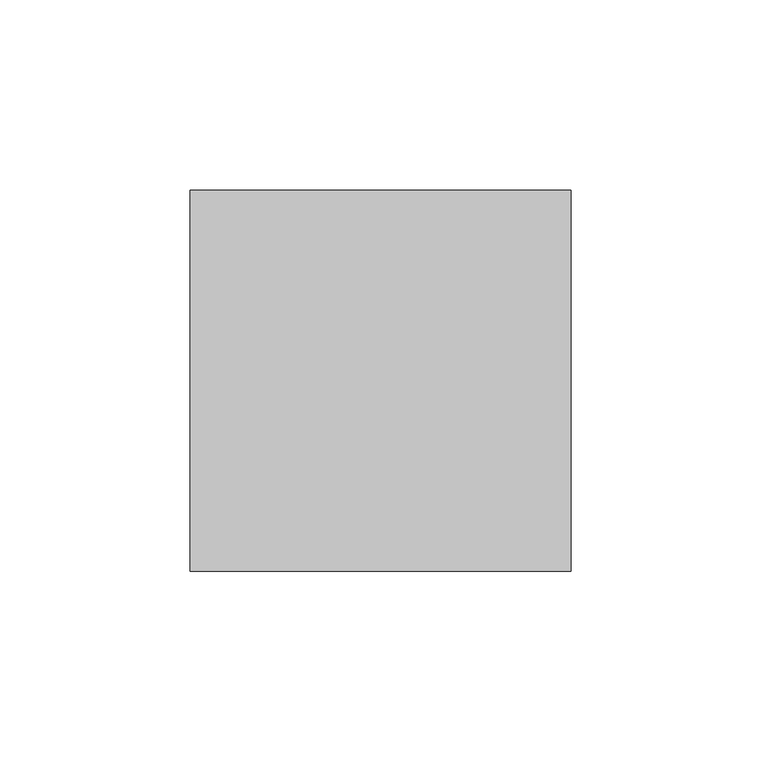
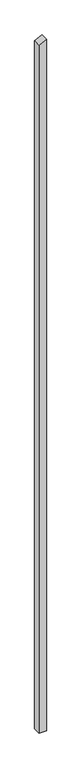
"""IFC4 building model written with IfcOpenShell, lengths in millimetres: column geometry, Holzstütze 159606 : Holzstütze 159606."""

import ifcopenshell
import ifcopenshell.guid

model = None  # the IFC model being written
_history = None  # IfcOwnerHistory: only IFC2X3 demands one
_inside = {}  # id of a spatial element -> (the spatial element, [elements in it])
_under = {}  # id of a project, library or spatial element -> (it, [spatial elements below it])
_declared = {}  # id of a project -> (the project, [libraries it declares])
_typed = {}  # id of a type object -> (the type object, [elements of that type])
_made_of = {}  # id of a material, layer set ... -> (it, [elements and type objects made of it])


def new_model(schema):
    """Start an empty IFC model of exactly this schema.

    Asked for "IFC4X3", IfcOpenShell would pick the latest addendum, in which some entities
    have other attributes; the version numbers below select the first issue.
    IFC2X3 requires an IfcOwnerHistory on every rooted entity: one is made here for all.
    """
    global model, _history
    if schema == "IFC4X3":
        model = ifcopenshell.file(schema_version=(4, 3, 0, 0))
    else:
        model = ifcopenshell.file(schema=schema)
    _inside.clear()
    _under.clear()
    _declared.clear()
    _typed.clear()
    _made_of.clear()
    _history = None
    if model.schema == "IFC2X3":
        org = make("IfcOrganization", Name="unknown")
        user = make(
            "IfcPersonAndOrganization",
            ThePerson=make("IfcPerson", FamilyName="unknown"),
            TheOrganization=org,
        )
        app = make(
            "IfcApplication",
            ApplicationDeveloper=org,
            Version="unknown",
            ApplicationFullName="unknown",
            ApplicationIdentifier="unknown",
        )
        _history = make(
            "IfcOwnerHistory",
            OwningUser=user,
            OwningApplication=app,
            ChangeAction="ADDED",
            CreationDate=0,
        )
    return model


def make(cls, **values):
    """One entity of the class cls with the attributes given. An attribute that is None is left unset."""
    return model.create_entity(
        cls, **{name: value for name, value in values.items() if value is not None}
    )


def rooted(cls, **values):
    """An entity with a GlobalId (a new one), such as an element, a storey or a relation."""
    return make(cls, GlobalId=ifcopenshell.guid.new(), OwnerHistory=_history, **values)


def si_unit(unit_type, name, prefix=None):
    """IfcSIUnit, for example si_unit("LENGTHUNIT", "METRE", prefix="MILLI")."""
    return make("IfcSIUnit", UnitType=unit_type, Prefix=prefix, Name=name)


def assignment(units):
    """IfcUnitAssignment: the units of a project."""
    return None if units is None else make("IfcUnitAssignment", Units=units)


def point(xyz):
    """IfcCartesianPoint."""
    return None if xyz is None else make("IfcCartesianPoint", Coordinates=xyz)


def direction(xyz):
    """IfcDirection."""
    return None if xyz is None else make("IfcDirection", DirectionRatios=xyz)


def frame(location, z_axis=None, x_axis=None):
    """IfcAxis2Placement3D, a coordinate frame: its origin and axes. An axis left out is left unset."""
    return make(
        "IfcAxis2Placement3D",
        Location=point(location),
        Axis=direction(z_axis),
        RefDirection=direction(x_axis),
    )


def origin():
    """The frame at (0, 0, 0) with its axes left unset."""
    return frame((0.0, 0.0, 0.0))


def place(relative_to, where):
    """IfcLocalPlacement: puts the frame where relative to a parent placement (None: the world)."""
    return make(
        "IfcLocalPlacement", PlacementRelTo=relative_to, RelativePlacement=where
    )


def context(
    kind, dimensions, precision=None, world=None, true_north=None, identifier=None
):
    """IfcGeometricRepresentationContext, for example the 3D "Model" context."""
    return make(
        "IfcGeometricRepresentationContext",
        ContextIdentifier=identifier,
        ContextType=kind,
        CoordinateSpaceDimension=dimensions,
        Precision=precision,
        WorldCoordinateSystem=world,
        TrueNorth=true_north,
    )


def project(units=None, contexts=None):
    """IfcProject with its units and contexts."""
    return rooted(
        "IfcProject",
        Name="project",
        RepresentationContexts=contexts,
        UnitsInContext=assignment(units),
    )


def spatial(cls, under=None, at=None, **own):
    """A site, building, storey or space (cls), placed at a placement, below another one or the project."""
    s = rooted(cls, ObjectPlacement=at, **own)
    if under is not None:
        _under.setdefault(under.id(), (under, []))[1].append(s)
    return s


def polyline(points):
    """IfcPolyline through the points."""
    return make("IfcPolyline", Points=[point(p) for p in points])


def outline(outer, holes=None, kind="AREA"):
    """IfcArbitraryClosedProfileDef: a profile drawn as a closed curve; with holes, ...WithVoids."""
    if holes is None:
        return make("IfcArbitraryClosedProfileDef", ProfileType=kind, OuterCurve=outer)
    return make(
        "IfcArbitraryProfileDefWithVoids",
        ProfileType=kind,
        OuterCurve=outer,
        InnerCurves=holes,
    )


def extrude(swept, where, along, depth):
    """IfcExtrudedAreaSolid: the profile swept, set in the frame where, extruded along a direction by depth."""
    return make(
        "IfcExtrudedAreaSolid",
        SweptArea=swept,
        Position=where,
        ExtrudedDirection=direction(along),
        Depth=depth,
    )


def shape(context_of_items, identifier, shape_type, items):
    """IfcShapeRepresentation: the items that make up one representation, for example the "Body"."""
    return make(
        "IfcShapeRepresentation",
        ContextOfItems=context_of_items,
        RepresentationIdentifier=identifier,
        RepresentationType=shape_type,
        Items=items,
    )


def source(mapping_origin, context_of_items, identifier, shape_type, items):
    """IfcRepresentationMap: a shape defined once, which mapped items show again and again."""
    return make(
        "IfcRepresentationMap",
        MappingOrigin=mapping_origin,
        MappedRepresentation=shape(context_of_items, identifier, shape_type, items),
    )


def transform(
    local_origin,
    x_axis=None,
    y_axis=None,
    z_axis=None,
    scale=None,
    scale2=None,
    scale3=None,
    uniform=True,
):
    """IfcCartesianTransformationOperator3D, or its non-uniform kind. x_axis, y_axis, z_axis: its Axis1, 2, 3."""
    if uniform:
        return make(
            "IfcCartesianTransformationOperator3D",
            Axis1=direction(x_axis),
            Axis2=direction(y_axis),
            LocalOrigin=point(local_origin),
            Scale=scale,
            Axis3=direction(z_axis),
        )
    return make(
        "IfcCartesianTransformationOperator3DnonUniform",
        Axis1=direction(x_axis),
        Axis2=direction(y_axis),
        LocalOrigin=point(local_origin),
        Scale=scale,
        Axis3=direction(z_axis),
        Scale2=scale2,
        Scale3=scale3,
    )


def mapped(mapping_source, mapping_target):
    """IfcMappedItem: shows the shape of a source again, moved by a transform."""
    return make(
        "IfcMappedItem", MappingSource=mapping_source, MappingTarget=mapping_target
    )


def made_of(thing, what):
    """Note that an element or type object is made of a material, layer set ...; save() writes the relation."""
    if what is not None:
        _made_of.setdefault(what.id(), (what, []))[1].append(thing)
    return thing


def element(
    cls,
    number,
    at=None,
    inside=None,
    cuts=None,
    type_object=None,
    material=None,
    context=None,
    identifier="Body",
    shape_type=None,
    held_by="IfcProductDefinitionShape",
    body=None,
    shapes=None,
    **own,
):
    """One element of the class cls, such as IfcWall. Its Tag is "e" and its number.

    at: its placement. inside: the storey or other place that contains it. cuts: it is an
    opening in that element (IfcRelVoidsElement). A single representation is given by context,
    identifier, shape_type and body (its items); several are given by shapes. held_by: the class
    of the entity that holds the representations. save() writes the other relations.
    """
    e = rooted(cls, Tag="e%d" % number, ObjectPlacement=at, **own)
    if body is not None:
        shapes = [shape(context, identifier, shape_type, body)]
    if shapes is not None:
        e.Representation = make(held_by, Representations=shapes)
    if inside is not None:
        _inside.setdefault(inside.id(), (inside, []))[1].append(e)
    if cuts is not None:
        rooted(
            "IfcRelVoidsElement", RelatingBuildingElement=cuts, RelatedOpeningElement=e
        )
    if type_object is not None:
        _typed.setdefault(type_object.id(), (type_object, []))[1].append(e)
    return made_of(e, material)


def aggregate(whole, parts):
    """IfcRelAggregates: a whole, such as a stair, and the parts it consists of."""
    return rooted("IfcRelAggregates", RelatingObject=whole, RelatedObjects=parts)


def save(model, path):
    """Write the relations noted so far, then the file.

    IfcRelAggregates (storeys below a building ...), IfcRelContainedInSpatialStructure (elements
    in a storey), IfcRelDefinesByType, IfcRelAssociatesMaterial and IfcRelDeclares: one each for
    every whole, place, type object, material and project.
    """
    for whole, parts in _under.values():
        aggregate(whole, parts)
    for where, things in _inside.values():
        rooted(
            "IfcRelContainedInSpatialStructure",
            RelatedElements=things,
            RelatingStructure=where,
        )
    for kind, things in _typed.values():
        rooted("IfcRelDefinesByType", RelatedObjects=things, RelatingType=kind)
    for what, things in _made_of.values():
        rooted("IfcRelAssociatesMaterial", RelatedObjects=things, RelatingMaterial=what)
    for by, libraries in _declared.values():
        rooted("IfcRelDeclares", RelatingContext=by, RelatedDefinitions=libraries)
    model.write(path)


def column_6093a7db(model_context):
    return source(origin(), model_context, "Body", "SweptSolid", [
        extrude(outline(polyline([(-500.0, 163237.7593015), (-500.0, 163337.7593015), (9423.2455407, 163337.7593015), (9372.2929958, 163237.7593015), (-500.0, 163237.7593015)])), frame((0.0, 26981.9343946, 0.0), z_axis=(0.0, 1.0, 0.0), x_axis=(0.0, 0.0, 1.0)), (0.0, 0.0, 1.0), 100.0),
    ])


if __name__ == "__main__":
    model = new_model("IFC4")
    model_context = context("Model", 3, world=origin())
    ifc_project = project(units=[si_unit("LENGTHUNIT", "METRE", prefix="MILLI")], contexts=[model_context])
    site = spatial("IfcSite", under=ifc_project)
    building = spatial("IfcBuilding", under=site)
    placement = place(None, origin())
    column_shape = column_6093a7db(model_context)
    element("IfcColumn", 1, ObjectType="Holzstütze 159606 : Holzstütze 159606", at=placement, inside=building, context=model_context, shape_type="MappedRepresentation", body=[
        mapped(column_shape, transform((0.0, 0.0, 0.0), x_axis=(1.0, 0.0, 0.0), y_axis=(0.0, 1.0, 0.0), z_axis=(0.0, 0.0, 1.0))),
    ])
    save(model, "model.ifc")

# Revit data of these elements
# Type "Holzstütze 159606 : Holzstütze 159606"
#   Abrechnungsart = "m"
#   Allright_Bauteil_ID = "0152St 0000143460"
#   Bezeichnung = "Holzstütze"
#   Codetext = "ST-HOLZ\\"
#   Gewerk = "Zimmer- und Holzbauarbeiten"
#   Material = "Holz"
#   Objektname = "Stütze"
#   NameOverride = "Holzstütze"
#   Reference = "Holzstütze"
#   Status = "NEW"
#   ThermalTransmittance = 0.0000 BTU/(h·ft²·°F)
#   Roll = 0.00°
#   Slope = 0.00°
#   2D Interaktion = yes
#   IsExternal = yes
#   LoadBearing = yes
# Element 1 (IfcColumn, "Holzstütze 159606 : Holzstütze 159606")
#   Materials on its faces: "holzschalung"
# Materials
#   "holzschalung": class "Unassigned", colour RGB 128 128 128, transparency 0
